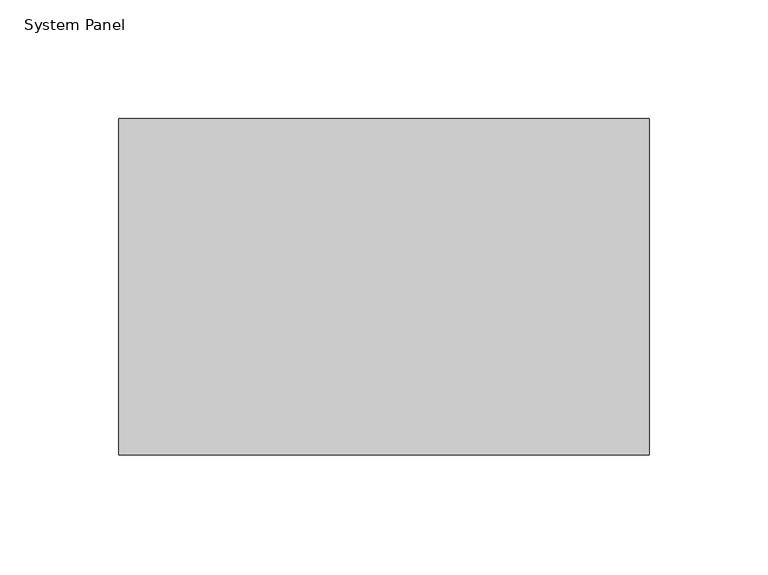
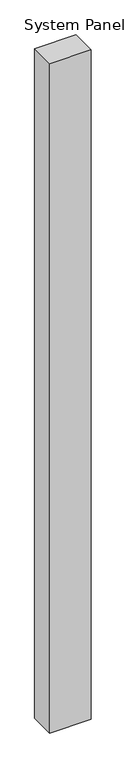
"""IFC4 building model written with IfcOpenShell, lengths in millimetres: plate geometry, System Panel : NLRS_21_CWP_hsb-vulling minerale wol 142 _gen_rsf."""

import ifcopenshell
import ifcopenshell.guid

model = None  # the IFC model being written
_history = None  # IfcOwnerHistory: only IFC2X3 demands one
_inside = {}  # id of a spatial element -> (the spatial element, [elements in it])
_under = {}  # id of a project, library or spatial element -> (it, [spatial elements below it])
_declared = {}  # id of a project -> (the project, [libraries it declares])
_typed = {}  # id of a type object -> (the type object, [elements of that type])
_made_of = {}  # id of a material, layer set ... -> (it, [elements and type objects made of it])


def new_model(schema):
    """Start an empty IFC model of exactly this schema.

    Asked for "IFC4X3", IfcOpenShell would pick the latest addendum, in which some entities
    have other attributes; the version numbers below select the first issue.
    IFC2X3 requires an IfcOwnerHistory on every rooted entity: one is made here for all.
    """
    global model, _history
    if schema == "IFC4X3":
        model = ifcopenshell.file(schema_version=(4, 3, 0, 0))
    else:
        model = ifcopenshell.file(schema=schema)
    _inside.clear()
    _under.clear()
    _declared.clear()
    _typed.clear()
    _made_of.clear()
    _history = None
    if model.schema == "IFC2X3":
        org = make("IfcOrganization", Name="unknown")
        user = make(
            "IfcPersonAndOrganization",
            ThePerson=make("IfcPerson", FamilyName="unknown"),
            TheOrganization=org,
        )
        app = make(
            "IfcApplication",
            ApplicationDeveloper=org,
            Version="unknown",
            ApplicationFullName="unknown",
            ApplicationIdentifier="unknown",
        )
        _history = make(
            "IfcOwnerHistory",
            OwningUser=user,
            OwningApplication=app,
            ChangeAction="ADDED",
            CreationDate=0,
        )
    return model


def make(cls, **values):
    """One entity of the class cls with the attributes given. An attribute that is None is left unset."""
    return model.create_entity(
        cls, **{name: value for name, value in values.items() if value is not None}
    )


def rooted(cls, **values):
    """An entity with a GlobalId (a new one), such as an element, a storey or a relation."""
    return make(cls, GlobalId=ifcopenshell.guid.new(), OwnerHistory=_history, **values)


def si_unit(unit_type, name, prefix=None):
    """IfcSIUnit, for example si_unit("LENGTHUNIT", "METRE", prefix="MILLI")."""
    return make("IfcSIUnit", UnitType=unit_type, Prefix=prefix, Name=name)


def assignment(units):
    """IfcUnitAssignment: the units of a project."""
    return None if units is None else make("IfcUnitAssignment", Units=units)


def point(xyz):
    """IfcCartesianPoint."""
    return None if xyz is None else make("IfcCartesianPoint", Coordinates=xyz)


def direction(xyz):
    """IfcDirection."""
    return None if xyz is None else make("IfcDirection", DirectionRatios=xyz)


def frame(location, z_axis=None, x_axis=None):
    """IfcAxis2Placement3D, a coordinate frame: its origin and axes. An axis left out is left unset."""
    return make(
        "IfcAxis2Placement3D",
        Location=point(location),
        Axis=direction(z_axis),
        RefDirection=direction(x_axis),
    )


def origin():
    """The frame at (0, 0, 0) with its axes left unset."""
    return frame((0.0, 0.0, 0.0))


def origin_with_axes():
    """The frame at (0, 0, 0) with the z axis (0, 0, 1) and the x axis (1, 0, 0) written out."""
    return frame((0.0, 0.0, 0.0), z_axis=(0.0, 0.0, 1.0), x_axis=(1.0, 0.0, 0.0))


def place(relative_to, where):
    """IfcLocalPlacement: puts the frame where relative to a parent placement (None: the world)."""
    return make(
        "IfcLocalPlacement", PlacementRelTo=relative_to, RelativePlacement=where
    )


def context(
    kind, dimensions, precision=None, world=None, true_north=None, identifier=None
):
    """IfcGeometricRepresentationContext, for example the 3D "Model" context."""
    return make(
        "IfcGeometricRepresentationContext",
        ContextIdentifier=identifier,
        ContextType=kind,
        CoordinateSpaceDimension=dimensions,
        Precision=precision,
        WorldCoordinateSystem=world,
        TrueNorth=true_north,
    )


def project(units=None, contexts=None):
    """IfcProject with its units and contexts."""
    return rooted(
        "IfcProject",
        Name="project",
        RepresentationContexts=contexts,
        UnitsInContext=assignment(units),
    )


def spatial(cls, under=None, at=None, **own):
    """A site, building, storey or space (cls), placed at a placement, below another one or the project."""
    s = rooted(cls, ObjectPlacement=at, **own)
    if under is not None:
        _under.setdefault(under.id(), (under, []))[1].append(s)
    return s


def polyline(points):
    """IfcPolyline through the points."""
    return make("IfcPolyline", Points=[point(p) for p in points])


def outline(outer, holes=None, kind="AREA"):
    """IfcArbitraryClosedProfileDef: a profile drawn as a closed curve; with holes, ...WithVoids."""
    if holes is None:
        return make("IfcArbitraryClosedProfileDef", ProfileType=kind, OuterCurve=outer)
    return make(
        "IfcArbitraryProfileDefWithVoids",
        ProfileType=kind,
        OuterCurve=outer,
        InnerCurves=holes,
    )


def extrude(swept, where, along, depth):
    """IfcExtrudedAreaSolid: the profile swept, set in the frame where, extruded along a direction by depth."""
    return make(
        "IfcExtrudedAreaSolid",
        SweptArea=swept,
        Position=where,
        ExtrudedDirection=direction(along),
        Depth=depth,
    )


def shape(context_of_items, identifier, shape_type, items):
    """IfcShapeRepresentation: the items that make up one representation, for example the "Body"."""
    return make(
        "IfcShapeRepresentation",
        ContextOfItems=context_of_items,
        RepresentationIdentifier=identifier,
        RepresentationType=shape_type,
        Items=items,
    )


def source(mapping_origin, context_of_items, identifier, shape_type, items):
    """IfcRepresentationMap: a shape defined once, which mapped items show again and again."""
    return make(
        "IfcRepresentationMap",
        MappingOrigin=mapping_origin,
        MappedRepresentation=shape(context_of_items, identifier, shape_type, items),
    )


def transform(
    local_origin,
    x_axis=None,
    y_axis=None,
    z_axis=None,
    scale=None,
    scale2=None,
    scale3=None,
    uniform=True,
):
    """IfcCartesianTransformationOperator3D, or its non-uniform kind. x_axis, y_axis, z_axis: its Axis1, 2, 3."""
    if uniform:
        return make(
            "IfcCartesianTransformationOperator3D",
            Axis1=direction(x_axis),
            Axis2=direction(y_axis),
            LocalOrigin=point(local_origin),
            Scale=scale,
            Axis3=direction(z_axis),
        )
    return make(
        "IfcCartesianTransformationOperator3DnonUniform",
        Axis1=direction(x_axis),
        Axis2=direction(y_axis),
        LocalOrigin=point(local_origin),
        Scale=scale,
        Axis3=direction(z_axis),
        Scale2=scale2,
        Scale3=scale3,
    )


def mapped(mapping_source, mapping_target):
    """IfcMappedItem: shows the shape of a source again, moved by a transform."""
    return make(
        "IfcMappedItem", MappingSource=mapping_source, MappingTarget=mapping_target
    )


def made_of(thing, what):
    """Note that an element or type object is made of a material, layer set ...; save() writes the relation."""
    if what is not None:
        _made_of.setdefault(what.id(), (what, []))[1].append(thing)
    return thing


def element(
    cls,
    number,
    at=None,
    inside=None,
    cuts=None,
    type_object=None,
    material=None,
    context=None,
    identifier="Body",
    shape_type=None,
    held_by="IfcProductDefinitionShape",
    body=None,
    shapes=None,
    **own,
):
    """One element of the class cls, such as IfcWall. Its Tag is "e" and its number.

    at: its placement. inside: the storey or other place that contains it. cuts: it is an
    opening in that element (IfcRelVoidsElement). A single representation is given by context,
    identifier, shape_type and body (its items); several are given by shapes. held_by: the class
    of the entity that holds the representations. save() writes the other relations.
    """
    e = rooted(cls, Tag="e%d" % number, ObjectPlacement=at, **own)
    if body is not None:
        shapes = [shape(context, identifier, shape_type, body)]
    if shapes is not None:
        e.Representation = make(held_by, Representations=shapes)
    if inside is not None:
        _inside.setdefault(inside.id(), (inside, []))[1].append(e)
    if cuts is not None:
        rooted(
            "IfcRelVoidsElement", RelatingBuildingElement=cuts, RelatedOpeningElement=e
        )
    if type_object is not None:
        _typed.setdefault(type_object.id(), (type_object, []))[1].append(e)
    return made_of(e, material)


def aggregate(whole, parts):
    """IfcRelAggregates: a whole, such as a stair, and the parts it consists of."""
    return rooted("IfcRelAggregates", RelatingObject=whole, RelatedObjects=parts)


def save(model, path):
    """Write the relations noted so far, then the file.

    IfcRelAggregates (storeys below a building ...), IfcRelContainedInSpatialStructure (elements
    in a storey), IfcRelDefinesByType, IfcRelAssociatesMaterial and IfcRelDeclares: one each for
    every whole, place, type object, material and project.
    """
    for whole, parts in _under.values():
        aggregate(whole, parts)
    for where, things in _inside.values():
        rooted(
            "IfcRelContainedInSpatialStructure",
            RelatedElements=things,
            RelatingStructure=where,
        )
    for kind, things in _typed.values():
        rooted("IfcRelDefinesByType", RelatedObjects=things, RelatingType=kind)
    for what, things in _made_of.values():
        rooted("IfcRelAssociatesMaterial", RelatedObjects=things, RelatingMaterial=what)
    for by, libraries in _declared.values():
        rooted("IfcRelDeclares", RelatingContext=by, RelatedDefinitions=libraries)
    model.write(path)


def system_panel_59c625bf(model_context):
    return source(origin(), model_context, "Body", "SweptSolid", [
        extrude(outline(polyline([(111.9999998, -71.0), (-111.9999998, -71.0), (-111.9999998, 71.0), (111.9999998, 71.0), (111.9999998, -71.0)])), origin_with_axes(), (0.0, 0.0, 1.0), 3849.0),
    ])


if __name__ == "__main__":
    model = new_model("IFC4")
    model_context = context("Model", 3, world=origin())
    ifc_project = project(units=[si_unit("LENGTHUNIT", "METRE", prefix="MILLI")], contexts=[model_context])
    site = spatial("IfcSite", under=ifc_project)
    building = spatial("IfcBuilding", under=site)
    placement = place(None, origin())
    system_panel_shape = system_panel_59c625bf(model_context)
    element("IfcPlate", 1, ObjectType="System Panel : NLRS_21_CWP_hsb-vulling minerale wol 142 _gen_rsf", at=placement, inside=building, context=model_context, shape_type="MappedRepresentation", body=[
        mapped(system_panel_shape, transform((0.0, 0.0, 0.0), x_axis=(1.0, 0.0, 0.0), y_axis=(0.0, 1.0, 0.0), z_axis=(0.0, 0.0, 1.0))),
    ])
    save(model, "model.ifc")

# Revit data of these elements
# Type "System Panel : NLRS_21_CWP_hsb-vulling minerale wol 142 _gen_rsf"
#   Export Type to IFC As = "IfcWall"
#   Type IfcGUID = "07M7mRoiH1CR8m_RSKIwpC"
#   Assembly Code = "21.23"
# Element 1 (IfcPlate, "System Panel : NLRS_21_CWP_hsb-vulling minerale wol 142 _gen_rsf")
#   Materials on its faces: "NLRS_m1_isolatie minerale wol_gen_rsf"
# Materials
#   "NLRS_m1_isolatie minerale wol_gen_rsf": class "M - Anorganische materialen", colour RGB 200 200 140, transparency 0, Keynote = "m1", Manufacturer = "Revit Standards Foundation", URL = "www.revitstandards.org", Description = "isolatie minerale wol", Cost = 0
